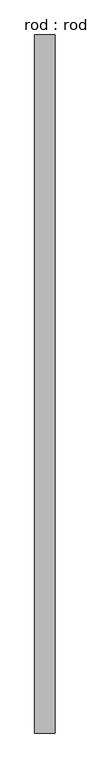
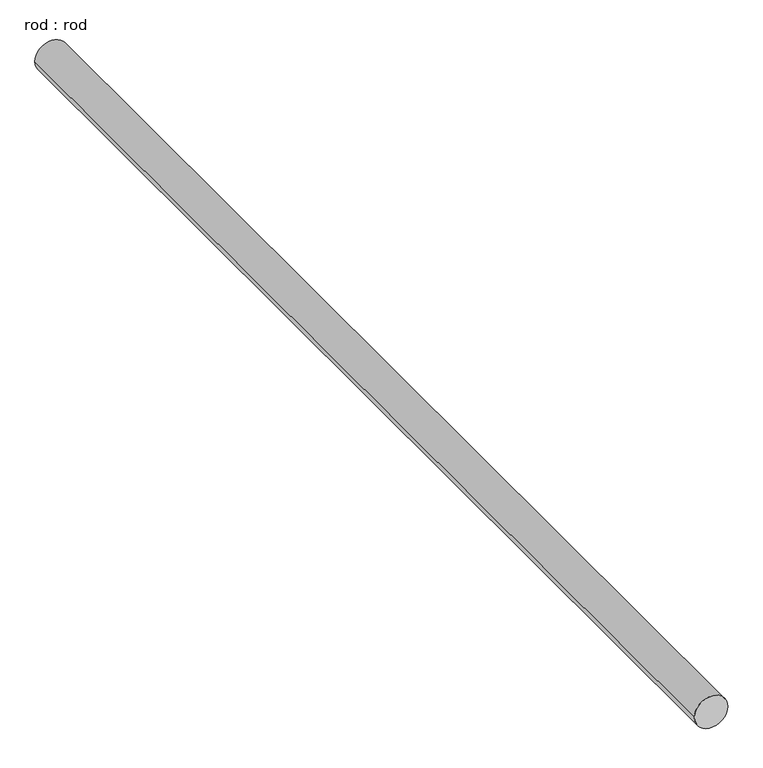
"""IFC4 building model written with IfcOpenShell, lengths in millimetres: proxy geometry, rod : rod."""

from ifc_helpers import new_model, si_unit, point, frame, frame_2d, origin, place, context, project, spatial, circle_curve, trimmed, segment, composite_curve, outline, extrude, source, transform, mapped, element, save


def rod_rod_5c4f7d59(model_context):
    return source(origin(), model_context, "Body", "SweptSolid", [
        extrude(outline(composite_curve([segment(trimmed(circle_curve(frame_2d((0.0108462, 0.0)), 200.0), [point((0.0108462, 200.0))], [point((0.0108462, -200.0))], False, "CARTESIAN"), True, "CONTINUOUS"), segment(trimmed(circle_curve(frame_2d((0.0108462, 0.0)), 200.0), [point((0.0108462, -200.0))], [point((0.0108462, 200.0))], False, "CARTESIAN"), True, "CONTINUOUS")], self_intersect=False)), frame((0.0, -2782.2713847, 0.0), z_axis=(0.0, 1.0, 0.0), x_axis=(0.0, 0.0, 1.0)), (0.0, 0.0, 1.0), 13750.0),
    ])


if __name__ == "__main__":
    model = new_model("IFC4")
    model_context = context("Model", 3, world=origin())
    ifc_project = project(units=[si_unit("LENGTHUNIT", "METRE", prefix="MILLI")], contexts=[model_context])
    site = spatial("IfcSite", under=ifc_project)
    building = spatial("IfcBuilding", under=site)
    placement = place(None, origin())
    rod_rod_shape = rod_rod_5c4f7d59(model_context)
    element("IfcBuildingElementProxy", 1, Name="rod : rod", ObjectType="rod : rod", at=placement, inside=building, context=model_context, shape_type="MappedRepresentation", body=[
        mapped(rod_rod_shape, transform((0.0, 0.0, 0.0), x_axis=(1.0, 0.0, 0.0), y_axis=(0.0, 1.0, 0.0), z_axis=(0.0, 0.0, 1.0))),
    ])
    save(model, "model.ifc")

# Revit data of these elements
# Type "rod : rod"
#   Default Elevation = 0
